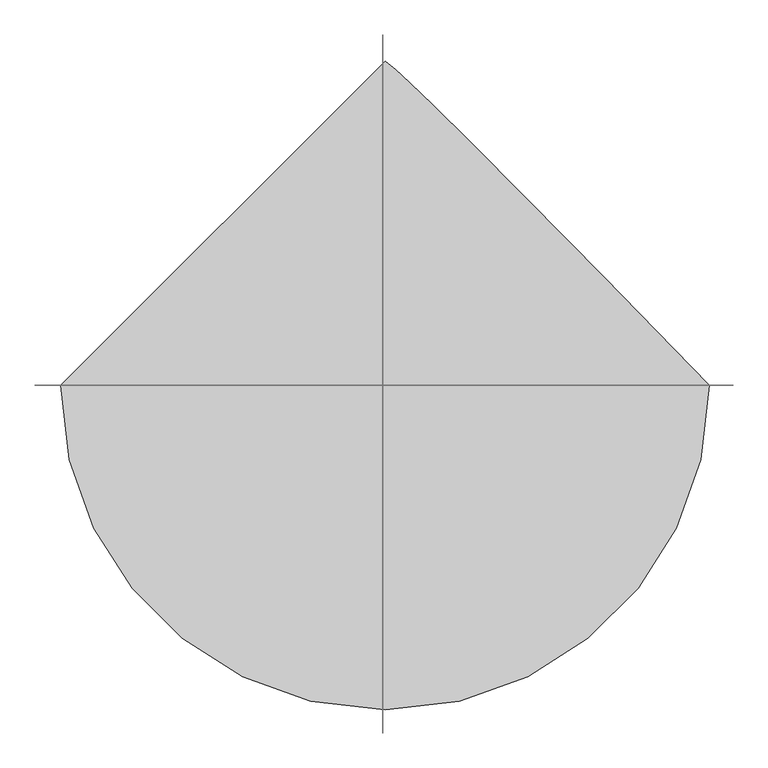
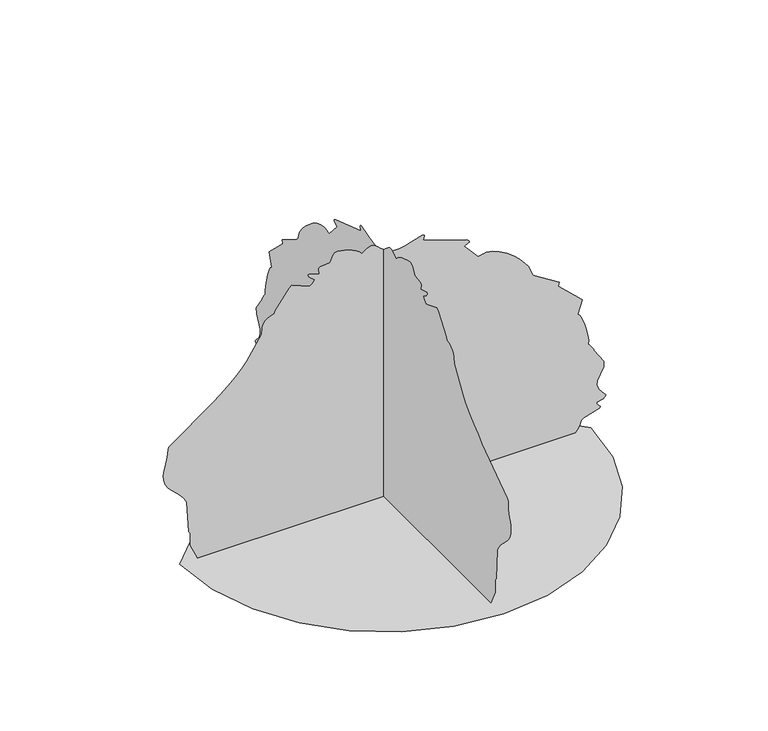
"""IFC4 building model written with IfcOpenShell, lengths in millimetres: proxy geometry, holly 26750 : holly 26750."""

from ifc_helpers import new_model, si_unit, origin, place, context, project, spatial, triangles, source, transform, mapped, element, save


def entourage_c51d7213(model_context):
    return source(origin(), model_context, "Body", "Tessellation", [
        triangles([(-948.1489574, 0.0, 0.0001584), (-923.0842083, -217.2530545, 0.0001584), (-851.6949612, -416.7657311, 0.0001584), (-739.7012884, -592.8207553, 0.0001584), (-592.8207553, -739.7012884, 0.0001584), (-416.7657311, -851.6949612, 0.0001584), (-217.2530545, -923.0816648, 0.0001584), (4.14e-05, -948.1489574, 0.0001584), (217.2530545, -923.0842083, 0.0001584), (416.7657311, -851.6949612, 0.0001584), (592.8207553, -739.7012884, 0.0001584), (739.7012884, -592.8207553, 0.0001584), (851.6949612, -416.7657311, 0.0001584), (923.0816648, -217.2530545, 0.0001584), (948.1489574, 8.29e-05, 0.0001584), (640.0215443, 316.0623576, 0.0001584), (411.5917374, 548.7669763, 0.0001584), (249.5753185, 712.0026157, 0.0001584), (140.6913579, 819.6655935, 0.0001584), (71.6559369, 885.64972, 0.0001584), (29.1863771, 923.8462257, 0.0001584), (-0.0001243, 948.1489574, 0.0001584), (-7.5086714, -195.1763861, 1267.2389282), (-7.5086714, -179.2483067, 1263.2994884), (-7.5086714, -162.0304078, 1257.8307816), (-7.5086714, -144.4787539, 1250.7569401), (-7.5086714, -127.5514259, 1242.0092182), (-7.5086714, -112.2047518, 1231.5139286), (-7.5086714, -99.3960405, 1219.1973839), (-7.5086714, -96.3241623, 1220.6731659), (-7.5086714, -91.1522123, 1224.4323841), (-7.5086714, -84.5334848, 1229.4921043), (-7.5086714, -77.1194751, 1234.8564571), (-7.5086714, -69.5642495, 1239.5377121), (-7.5086714, -62.5195578, 1242.5399998), (-7.5086714, -56.6381899, 1242.880386), (-7.5086714, -48.1497636, 1241.0642178), (-7.5086714, -38.0075433, 1235.3112259), (-7.5086714, -26.6616175, 1226.6954727), (-7.5086714, -14.5605495, 1216.2942181), (-7.5086714, -2.1549868, 1205.1816696), (-7.5086714, 10.1063292, 1194.4323984), (-7.5086714, 21.7735642, 1185.1233009), (-7.5086714, 44.9310738, 1181.1406225), (-7.5086714, 71.2939859, 1182.9871668), (-7.5086714, 98.7844045, 1188.6996088), (-7.5086714, 125.3246087, 1196.3018337), (-7.5086714, 178.4657237, 1210.777331), (-7.5086714, 184.0044481, 1210.1194496), (-7.5086714, 186.6691655, 1206.9444254), (-7.5086714, 187.1967314, 1202.1768385), (-7.5086714, 182.6755321, 1185.5170269), (-7.5086714, 383.1462716, 1117.5161631), (-7.5086714, 393.1767277, 1109.7361147), (-7.5086714, 395.0157143, 1105.6136919), (-7.5086714, 393.8879488, 1102.1694254), (-7.5086714, 390.6062814, 1099.2180067), (-7.5086714, 372.1277581, 1088.6871088), (-7.5086714, 435.2772466, 1017.1175674), (-7.5086714, 437.7283324, 1017.437606), (-7.5086714, 442.2698793, 1018.3037596), (-7.5086714, 448.2439333, 1019.5610229), (-7.5086714, 454.9825481, 1021.0621668), (-7.5086714, 461.822792, 1022.6598164), (-7.5086714, 468.1067471, 1024.2016554), (-7.5086714, 473.166431, 1025.537693), (-7.5086714, 502.5059555, 1020.5592905), (-7.5086714, 534.2381756, 1007.0464525), (-7.5086714, 566.6435014, 987.1252121), (-7.5086714, 598.0048865, 962.9266891), (-7.5086714, 626.6103716, 936.5792421), (-7.5086714, 650.7352798, 910.2089767), (-7.5086714, 668.6702316, 885.9468676), (-7.5086714, 686.5644882, 838.1898262), (-7.5086714, 809.9704004, 760.305772), (-7.5086714, 805.7591022, 743.4655935), (-7.5086714, 915.2203714, 638.2130791), (-7.5086714, 894.1714382, 575.0635906), (-7.5086714, 903.617664, 567.5579078), (-7.5086714, 914.1053232, 547.8068604), (-7.5086714, 924.5625338, 519.9684434), (-7.5086714, 933.9198841, 488.2006877), (-7.5086714, 941.1080355, 456.6564285), (-7.5086714, 945.0552509, 429.4962041), (-7.5086714, 944.6894302, 410.8729222), (-7.5086714, 947.6840876, 408.4091191), (-7.5086714, 951.631303, 403.9311221), (-7.5086714, 956.0813948, 398.0789357), (-7.5086714, 960.5872971, 391.4952533), (-7.5086714, 964.7020895, 384.820152), (-7.5086714, 967.971076, 378.6987597), (-7.5086714, 969.9497343, 373.7711535), (-7.5086714, 1015.9974323, 304.568855), (-7.5086714, 1014.0136871, 276.7279126), (-7.5086714, 984.4354053, 218.9253907), (-7.5086714, 983.4092325, 198.3142941), (-7.5086714, 995.1541552, 172.0712739), (-7.5086714, 1024.6817133, 137.2212117), (-7.5086714, 1022.9417759, 130.8493623), (-7.5086714, 1018.3139334, 126.0055809), (-7.5086714, 1011.6743677, 122.4462869), (-7.5086714, 982.5811581, 116.1709614), (-7.5086714, 982.5024565, 110.3304839), (-7.5086714, 984.7630743, 105.408982), (-7.5086714, 999.0657623, 90.4069817), (-7.5086714, 999.4214092, 86.700867), (-7.5086714, 994.9103474, 81.6175654), (-7.5086714, 922.3882479, 60.3801172), (-7.5086714, 911.0090733, 53.020719), (-7.5086714, 909.9524517, 45.2163171), (-7.5086714, 907.5597198, 37.5411996), (-7.5086714, 904.0596428, 29.9740312), (-7.5086714, 899.6679777, 22.4928926), (-7.5086714, 894.6082575, 15.0766517), (-7.5086714, 889.1066311, 7.7034389), (-7.5086714, 883.3814718, 0.3517747), (-7.5086714, -857.0696331, 0.0), (-7.5086714, -890.8821041, 74.070715), (-7.5086714, -890.8821041, 133.011158), (-7.5086714, -897.8544256, 142.0888652), (-7.5086714, -906.9323599, 288.2569691), (-7.5086714, -918.2785423, 310.329568), (-7.5086714, -934.7885084, 330.547956), (-7.5086714, -954.1814381, 349.7579753), (-7.5086714, -974.171279, 368.8105187), (-7.5086714, -992.4846233, 388.5513923), (-7.5086714, -1006.8356369, 409.831525), (-7.5086714, -1014.945825, 433.5017735), (-7.5086714, -1016.3835279, 454.0351496), (-7.5086714, -1014.4251446, 473.0826061), (-7.5086714, -1010.2722731, 490.9768991), (-7.5086714, -1005.1338512, 508.0558711), (-7.5086714, -996.7289864, 541.0987307), (-7.5086714, -993.7038076, 576.6841312), (-7.5086714, -989.7007816, 586.0592494), (-7.5086714, -986.7239285, 589.1733035), (-7.5086714, -784.7202702, 733.315777), (-7.5086714, -753.8211388, 759.3609169), (-7.5086714, -719.0663561, 789.2566938), (-7.5086714, -684.3724709, 820.8568726), (-7.5086714, -653.6486195, 852.0099129), (-7.5086714, -630.8089525, 880.5697248), (-7.5086714, -562.4982239, 987.6459652), (-7.5086714, -559.6966144, 1020.7294109), (-7.5086714, -555.292232, 1034.4301735), (-7.5086714, -548.0761027, 1046.0812065), (-7.5086714, -537.4512789, 1055.5756851), (-7.5086714, -522.8132552, 1062.7994448), (-7.5086714, -503.5575265, 1067.6381756), (-7.5086714, -500.3495101, 1081.6894255), (-7.5086714, -435.3305863, 1167.4931997), (-7.5086714, -423.5678596, 1177.0969013), (-7.5086714, -339.3668581, 1143.4165443), (-7.5086714, -336.5372706, 1144.8643484), (-7.5086714, -333.0320704, 1147.7802315), (-7.5086714, -329.2195487, 1151.7172005), (-7.5086714, -318.3178522, 1168.6768484), (-7.5086714, -338.9502774, 1184.7296476), (-7.5086714, -344.6017857, 1191.1278763), (-7.5086714, -347.962191, 1197.2136967), (-7.5086714, -347.7869473, 1202.3572054), (-7.5086714, -343.1539816, 1204.0539042), (-7.5086714, -297.2663574, 1189.7283251), (-7.5086714, -299.3516952, 1212.9287258), (-7.5086714, -298.767483, 1216.5431128), (-7.5086714, -297.2663574, 1219.1973839), (-7.5086714, -292.6613332, 1221.3539383), (-7.5086714, -249.2443431, 1226.9900768), (-7.5086714, -246.747021, 1227.6175095), (-7.5086714, -231.2268564, 1258.3413609), (-7.5086714, -224.3381235, 1265.7124226), (-7.5086714, -216.7902557, 1269.9999516), (-7.5086714, -208.8568192, 1269.717992), (-202.6848849, -7.94e-05, 1267.2389282), (-186.7567873, -7.9e-05, 1263.2994884), (-169.5388885, -7.87e-05, 1257.8307816), (-151.9872436, -7.84e-05, 1250.7569401), (-135.0599247, -7.8e-05, 1242.0092182), (-119.7134959, -7.75e-05, 1231.5139286), (-106.9047846, -7.68e-05, 1219.1973839), (-103.8329063, -7.69e-05, 1220.6731659), (-98.6609655, -7.7e-05, 1224.4323841), (-92.0419745, -7.73e-05, 1229.4921043), (-84.6279739, -7.75e-05, 1234.8564571), (-77.0729936, -7.78e-05, 1239.5377121), (-70.0280521, -7.8e-05, 1242.5399998), (-64.1469339, -7.83e-05, 1242.880386), (-55.6582578, -7.75e-05, 1241.0642178), (-45.5160353, -7.69e-05, 1235.3112259), (-34.1701118, -7.64e-05, 1226.6954727), (-22.0691448, -7.6e-05, 1216.2942181), (-9.6635817, -7.56e-05, 1205.1816696), (2.5977342, -7.53e-05, 1194.4323984), (14.26497, -7.48e-05, 1185.1233009), (37.4223274, -7.46e-05, 1181.1406225), (63.7852418, -7.46e-05, 1182.9871668), (91.2759148, -7.49e-05, 1188.6996088), (117.816119, -7.54e-05, 1196.3018337), (170.9569705, -7.63e-05, 1210.777331), (176.4956949, -7.62e-05, 1210.1194496), (179.1604124, -7.6e-05, 1206.9444254), (179.6879783, -7.57e-05, 1202.1768385), (175.1670333, -7.48e-05, 1185.5170269), (375.6380453, -7.06e-05, 1117.5161631), (385.6685014, -7.03e-05, 1109.7361147), (387.5074516, -7.02e-05, 1105.6136919), (386.3797225, -7e-05, 1102.1694254), (383.0980187, -6.98e-05, 1099.2180067), (364.6195318, -6.91e-05, 1088.6871088), (427.7690203, -6.48e-05, 1017.1175674), (430.2201061, -6.48e-05, 1017.437606), (434.7616167, -6.49e-05, 1018.3037596), (440.735707, -6.5e-05, 1019.5610229), (447.4743218, -6.5e-05, 1021.0621668), (454.3145293, -6.51e-05, 1022.6598164), (460.5984844, -6.52e-05, 1024.2016554), (465.6581683, -6.53e-05, 1025.537693), (494.9977292, -6.5e-05, 1020.5592905), (526.7299493, -6.42e-05, 1007.0464525), (559.1352751, -6.3e-05, 987.1252121), (590.4966239, -6.16e-05, 962.9266891), (619.0995655, -6e-05, 936.5792421), (643.2270172, -5.84e-05, 910.2089767), (661.161969, -5.7e-05, 885.9468676), (679.0537548, -5.41e-05, 838.1898262), (802.4621378, -4.95e-05, 760.305772), (798.2508396, -4.85e-05, 743.4655935), (907.7121815, -4.22e-05, 638.2156225), (886.6606321, -3.85e-05, 575.0635906), (896.1094013, -3.8e-05, 567.5579078), (906.5970606, -3.68e-05, 547.8068604), (917.0542711, -3.52e-05, 519.9684434), (926.4116215, -3.33e-05, 488.2006877), (933.5973021, -3.14e-05, 456.6564285), (937.5444448, -2.98e-05, 429.4962041), (937.1812403, -2.87e-05, 410.8729222), (940.1758976, -2.85e-05, 408.4091191), (944.1230404, -2.83e-05, 403.9311221), (948.5731321, -2.79e-05, 398.0789357), (953.0791071, -2.75e-05, 391.4952533), (957.1913561, -2.71e-05, 384.820152), (960.462886, -2.68e-05, 378.6987597), (962.4415443, -2.65e-05, 373.7711535), (1008.4891697, -2.23e-05, 304.568855), (1006.5054245, -2.07e-05, 276.7279126), (976.9271427, -1.72e-05, 218.9253907), (975.9009699, -1.6e-05, 198.3142941), (987.6459652, -1.44e-05, 172.0712739), (1017.1734507, -1.24e-05, 137.2212117), (1015.4335133, -1.2e-05, 130.8493623), (1010.8056707, -1.17e-05, 126.0058353), (1004.1661051, -1.15e-05, 122.4462869), (975.0729681, -1.11e-05, 116.1712157), (974.9941938, -1.11e-05, 110.3304839), (977.2548117, -1.08e-05, 105.408982), (991.5575724, -9.4e-06, 90.407236), (991.9131466, -9.3e-06, 86.700867), (987.4020847, -9.1e-06, 81.6175654), (914.8800579, -7.5e-06, 60.3801172), (903.5008106, -7.3e-06, 53.020719), (902.4441891, -7.5e-06, 45.2163171), (900.0515299, -7.5e-06, 37.5411996), (896.5488367, -7.3e-06, 29.9740312), (892.1597151, -6.9e-06, 22.4929448), (887.1000675, -6.5e-06, 15.0767278), (881.5984411, -6e-06, 7.7034894), (875.8732819, -5.5e-06, 0.3518408), (-864.5778957, -4.1e-06, 6.72e-05), (-898.3903667, -8.6e-06, 74.0709693), (-898.3903667, -1.21e-05, 133.011158), (-905.3626156, -1.26e-05, 142.0888652), (-914.4406225, -2.14e-05, 288.2569691), (-925.7893484, -2.27e-05, 310.3321115), (-942.296771, -2.39e-05, 330.547956), (-961.6897007, -2.5e-05, 349.7579753), (-981.6820124, -2.62e-05, 368.8105187), (-999.992886, -2.73e-05, 388.5513923), (-1014.3438995, -2.86e-05, 409.831525), (-1022.4540876, -3e-05, 433.5017735), (-1023.8917179, -3.12e-05, 454.0351496), (-1021.9334072, -3.24e-05, 473.0826061), (-1017.7805357, -3.34e-05, 490.9768991), (-1012.6421139, -3.45e-05, 508.0558711), (-1004.237249, -3.64e-05, 541.0987307), (-1001.2146137, -3.86e-05, 576.6841312), (-997.2090443, -3.92e-05, 586.0592494), (-994.2347345, -3.94e-05, 589.1733035), (-792.2285328, -4.83e-05, 733.315777), (-761.3294014, -5.01e-05, 759.3609169), (-726.5746187, -5.21e-05, 789.2566938), (-691.8807335, -5.41e-05, 820.8568726), (-661.1568821, -5.59e-05, 852.0099129), (-638.3172152, -5.74e-05, 880.5697248), (-570.0064502, -6.3e-05, 987.6459652), (-567.2048407, -6.5e-05, 1020.7294109), (-562.8004947, -6.58e-05, 1034.4301735), (-555.584329, -6.65e-05, 1046.0812065), (-544.9595052, -6.71e-05, 1055.5756851), (-530.3215178, -6.75e-05, 1062.7994448), (-511.0682962, -6.78e-05, 1067.6381756), (-507.8577364, -6.87e-05, 1081.6894255), (-442.8413561, -7.38e-05, 1167.4931997), (-431.0760859, -7.43e-05, 1177.0969013), (-346.8750844, -7.23e-05, 1143.4165443), (-344.0455333, -7.24e-05, 1144.8643484), (-340.540333, -7.26e-05, 1147.7802315), (-336.727775, -7.28e-05, 1151.7172005), (-325.8261148, -7.38e-05, 1168.6768484), (-346.4585401, -7.48e-05, 1184.7296476), (-352.110012, -7.51e-05, 1191.1278763), (-355.4704536, -7.55e-05, 1197.2136967), (-355.2951736, -7.58e-05, 1202.3572054), (-350.6622442, -7.57e-05, 1204.0539042), (-304.7771271, -7.51e-05, 1189.7283251), (-306.8599397, -7.63e-05, 1212.9287258), (-306.2757457, -7.65e-05, 1216.5431128), (-304.7771271, -7.68e-05, 1219.1973839), (-300.1695595, -7.68e-05, 1221.3539383), (-256.7533506, -7.73e-05, 1226.9900768), (-254.2565372, -7.74e-05, 1227.6175095), (-238.7353552, -7.86e-05, 1258.3413609), (-231.8468767, -7.9e-05, 1265.7124226), (-224.2990089, -7.94e-05, 1269.9999516), (-216.3655724, -7.99e-05, 1269.717992)], [[21, 22, 1], [20, 21, 1], [19, 20, 1], [18, 19, 1], [17, 18, 1], [17, 1, 2], [17, 2, 3], [17, 3, 4], [16, 17, 4], [16, 4, 5], [16, 5, 6], [16, 6, 7], [16, 7, 8], [16, 8, 9], [16, 9, 10], [16, 10, 11], [16, 11, 12], [15, 16, 12], [14, 15, 12], [13, 14, 12], [74, 75, 76], [160, 161, 162], [116, 117, 118], [116, 118, 119], [76, 77, 78], [159, 160, 162], [158, 159, 162], [157, 158, 162], [157, 162, 163], [151, 152, 153], [115, 116, 119], [114, 115, 119], [113, 114, 119], [112, 113, 119], [111, 112, 119], [110, 111, 119], [109, 110, 119], [97, 98, 99], [97, 99, 100], [97, 100, 101], [97, 101, 102], [109, 119, 120], [109, 120, 121], [109, 121, 122], [105, 106, 107], [104, 105, 107], [104, 107, 108], [103, 104, 108], [150, 151, 153], [149, 150, 153], [48, 49, 50], [48, 50, 51], [48, 51, 52], [47, 48, 52], [109, 122, 123], [54, 55, 56], [54, 56, 57], [53, 54, 57], [53, 57, 58], [52, 53, 58], [108, 109, 123], [102, 103, 108], [92, 93, 94], [92, 94, 95], [96, 97, 102], [96, 102, 108], [96, 108, 123], [95, 96, 123], [92, 95, 123], [91, 92, 123], [90, 91, 123], [89, 90, 123], [88, 89, 123], [87, 88, 123], [86, 87, 123], [85, 86, 123], [84, 85, 123], [83, 84, 123], [82, 83, 123], [81, 82, 123], [80, 81, 123], [79, 80, 123], [78, 79, 123], [76, 78, 123], [74, 76, 123], [73, 74, 123], [72, 73, 123], [71, 72, 123], [70, 71, 123], [69, 70, 123], [68, 69, 123], [67, 68, 123], [66, 67, 123], [65, 66, 123], [64, 65, 123], [63, 64, 123], [62, 63, 123], [61, 62, 123], [60, 61, 123], [59, 60, 123], [58, 59, 123], [52, 58, 123], [47, 52, 123], [46, 47, 123], [45, 46, 123], [44, 45, 123], [43, 44, 123], [42, 43, 123], [41, 42, 123], [40, 41, 123], [39, 40, 123], [38, 39, 123], [37, 38, 123], [36, 37, 123], [35, 36, 123], [34, 35, 123], [33, 34, 123], [32, 33, 123], [31, 32, 123], [30, 31, 123], [29, 30, 123], [29, 123, 124], [28, 29, 124], [27, 28, 124], [26, 27, 124], [25, 26, 124], [24, 25, 124], [23, 24, 124], [173, 23, 124], [173, 124, 125], [173, 125, 126], [165, 166, 167], [164, 165, 167], [163, 164, 167], [163, 167, 168], [171, 172, 173], [170, 171, 173], [169, 170, 173], [169, 173, 126], [168, 169, 126], [168, 126, 127], [168, 127, 128], [168, 128, 129], [168, 129, 130], [168, 130, 131], [168, 131, 132], [145, 146, 147], [145, 147, 148], [144, 145, 148], [144, 148, 149], [143, 144, 149], [143, 149, 153], [142, 143, 153], [134, 135, 136], [133, 134, 136], [133, 136, 137], [132, 133, 137], [142, 153, 154], [156, 157, 163], [156, 163, 168], [141, 142, 154], [132, 137, 138], [132, 138, 139], [141, 154, 155], [140, 141, 155], [155, 156, 168], [155, 168, 132], [140, 155, 132], [140, 132, 139], [225, 226, 227], [311, 312, 313], [267, 268, 269], [267, 269, 270], [227, 228, 229], [310, 311, 313], [309, 310, 313], [308, 309, 313], [308, 313, 314], [302, 303, 304], [266, 267, 270], [265, 266, 270], [264, 265, 270], [263, 264, 270], [262, 263, 270], [261, 262, 270], [260, 261, 270], [248, 249, 250], [248, 250, 251], [248, 251, 252], [248, 252, 253], [260, 270, 271], [260, 271, 272], [260, 272, 273], [256, 257, 258], [255, 256, 258], [255, 258, 259], [254, 255, 259], [301, 302, 304], [300, 301, 304], [199, 200, 201], [199, 201, 202], [199, 202, 203], [198, 199, 203], [260, 273, 274], [205, 206, 207], [205, 207, 208], [204, 205, 208], [204, 208, 209], [203, 204, 209], [259, 260, 274], [253, 254, 259], [243, 244, 245], [243, 245, 246], [247, 248, 253], [247, 253, 259], [247, 259, 274], [246, 247, 274], [243, 246, 274], [242, 243, 274], [241, 242, 274], [240, 241, 274], [239, 240, 274], [238, 239, 274], [237, 238, 274], [236, 237, 274], [235, 236, 274], [234, 235, 274], [233, 234, 274], [232, 233, 274], [231, 232, 274], [230, 231, 274], [229, 230, 274], [227, 229, 274], [225, 227, 274], [224, 225, 274], [223, 224, 274], [222, 223, 274], [221, 222, 274], [220, 221, 274], [219, 220, 274], [218, 219, 274], [217, 218, 274], [216, 217, 274], [215, 216, 274], [214, 215, 274], [213, 214, 274], [212, 213, 274], [211, 212, 274], [210, 211, 274], [209, 210, 274], [203, 209, 274], [198, 203, 274], [197, 198, 274], [196, 197, 274], [195, 196, 274], [194, 195, 274], [193, 194, 274], [192, 193, 274], [191, 192, 274], [190, 191, 274], [189, 190, 274], [188, 189, 274], [187, 188, 274], [186, 187, 274], [185, 186, 274], [184, 185, 274], [183, 184, 274], [182, 183, 274], [181, 182, 274], [180, 181, 274], [180, 274, 275], [179, 180, 275], [178, 179, 275], [177, 178, 275], [176, 177, 275], [175, 176, 275], [174, 175, 275], [324, 174, 275], [324, 275, 276], [324, 276, 277], [316, 317, 318], [315, 316, 318], [314, 315, 318], [314, 318, 319], [322, 323, 324], [321, 322, 324], [320, 321, 324], [320, 324, 277], [319, 320, 277], [319, 277, 278], [319, 278, 279], [319, 279, 280], [319, 280, 281], [319, 281, 282], [319, 282, 283], [296, 297, 298], [296, 298, 299], [295, 296, 299], [295, 299, 300], [294, 295, 300], [294, 300, 304], [293, 294, 304], [285, 286, 287], [284, 285, 287], [284, 287, 288], [283, 284, 288], [293, 304, 305], [307, 308, 314], [307, 314, 319], [292, 293, 305], [283, 288, 289], [283, 289, 290], [292, 305, 306], [291, 292, 306], [306, 307, 319], [306, 319, 283], [291, 306, 283], [291, 283, 290]], closed=False),
    ])


if __name__ == "__main__":
    model = new_model("IFC4")
    model_context = context("Model", 3, world=origin())
    ifc_project = project(units=[si_unit("LENGTHUNIT", "METRE", prefix="MILLI")], contexts=[model_context])
    site = spatial("IfcSite", under=ifc_project)
    building = spatial("IfcBuilding", under=site)
    placement = place(None, origin())
    entourage_shape = entourage_c51d7213(model_context)
    element("IfcBuildingElementProxy", 1, Name="holly 26750 : holly 26750", ObjectType="holly 26750 : holly 26750", at=placement, inside=building, context=model_context, shape_type="MappedRepresentation", body=[
        mapped(entourage_shape, transform((0.0, 0.0, 0.0), x_axis=(1.0, 0.0, 0.0), y_axis=(0.0, 1.0, 0.0), z_axis=(0.0, 0.0, 1.0))),
    ])
    save(model, "model.ifc")

# Revit data of these elements
# Type "holly 26750 : holly 26750"
#   built-in parameter 1005195 = "RPC-16-FVGN-EMQ0-7PXJ-Q000-ST1L-LVER-AU"
#   Height = 0
